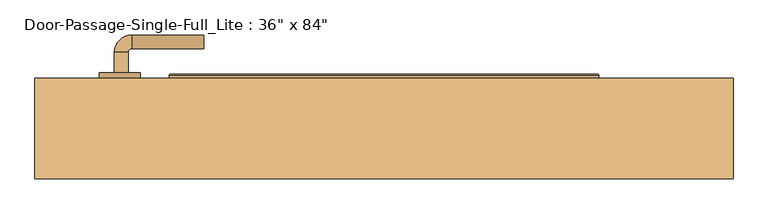
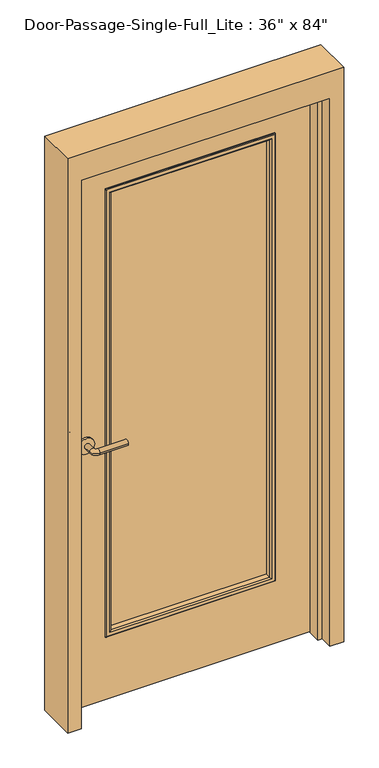
"""IFC4 building model written with IfcOpenShell, lengths in millimetres: door geometry."""

from ifc_helpers import new_model, si_unit, point, frame, frame_2d, origin, place, context, project, spatial, polyline, circle_curve, ellipse_curve, trimmed, segment, composite_curve, outline, extrude, faceted_brep, source, transform, mapped, element, save
from ifc_brep_helpers import plane_surface, cylinder_surface, revolved_surface, advanced_brep


def door_4a7c4c71(model_context):
    return source(origin(), model_context, "Body", "SolidModel", [
        advanced_brep(
        [(-392.190625, 23.75, 1016.0), (-372.190625, 23.75, 1016.0), (-372.190625, -6.25, 1016.0), (-392.190625, -6.25, 1016.0), (-367.190625, -11.25, 1016.0), (-367.190625, -31.25, 1016.0), (-262.190625, -31.25, 1016.0), (-262.190625, -11.25, 1016.0)],
        [
            (0, 1, circle_curve(frame((-382.190625, 23.75, 1016.0), z_axis=(0.0, 1.0, 0.0), x_axis=(1.0, 0.0, 0.0)), 10.0)),
            (1, 0, circle_curve(frame((-382.190625, 23.75, 1016.0), z_axis=(0.0, 1.0, 0.0), x_axis=(1.0, 0.0, 0.0)), 10.0)),
            (1, 2),
            (2, 3, circle_curve(frame((-382.190625, -6.25, 1016.0), z_axis=(0.0, 1.0, 0.0), x_axis=(1.0, 0.0, 0.0)), 10.0)),
            (3, 0),
            (3, 2, circle_curve(frame((-382.190625, -6.25, 1016.0), z_axis=(0.0, 1.0, 0.0), x_axis=(1.0, 0.0, 0.0)), 10.0)),
            (4, 5, circle_curve(frame((-367.190625, -21.25, 1016.0), z_axis=(-1.0, 0.0, 0.0), x_axis=(0.0, 1.0, 0.0)), 10.0)),
            (5, 3, circle_curve(frame((-367.190625, -6.25, 1016.0), z_axis=(0.0, 0.0, -1.0), x_axis=(-1.0, 0.0, 0.0)), 25.0)),
            (2, 4, circle_curve(frame((-367.190625, -6.25, 1016.0), z_axis=(0.0, 0.0, 1.0), x_axis=(-1.0, 0.0, 0.0)), 5.0)),
            (5, 4, circle_curve(frame((-367.190625, -21.25, 1016.0), z_axis=(-1.0, 0.0, 0.0), x_axis=(0.0, 1.0, 0.0)), 10.0)),
            (6, 7, circle_curve(frame((-262.190625, -21.25, 1016.0), z_axis=(1.0, 0.0, 0.0), x_axis=(0.0, 1.0, 0.0)), 10.0)),
            (7, 6, circle_curve(frame((-262.190625, -21.25, 1016.0), z_axis=(1.0, 0.0, 0.0), x_axis=(0.0, 1.0, 0.0)), 10.0)),
            (4, 7),
            (6, 5),
        ],
        [
            plane_surface(frame((-382.190625, 23.75, 1016.0), z_axis=(0.0, 1.0, 0.0), x_axis=(0.0, 0.0, 1.0))),
            cylinder_surface(frame((-382.190625, 23.75, 1016.0), z_axis=(0.0, 1.0, 0.0), x_axis=(1.0, 0.0, 0.0)), 10.0),
            revolved_surface(trimmed(ellipse_curve(frame((-382.190625, -6.25, 1016.0), z_axis=(0.0, -1.0, 0.0), x_axis=(1.0, 0.0, 0.0)), 10.0, 10.0), [point((-392.190625, -6.25, 1016.0))], [point((-372.190625, -6.25, 1016.0))], True, "CARTESIAN"), (-367.190625, -6.25, 1016.0), (0.0, 0.0, -1.0)),
            revolved_surface(trimmed(ellipse_curve(frame((-382.190625, -6.25, 1016.0), z_axis=(0.0, -1.0, 0.0), x_axis=(1.0, 0.0, 0.0)), 10.0, 10.0), [point((-372.190625, -6.25, 1016.0))], [point((-392.190625, -6.25, 1016.0))], True, "CARTESIAN"), (-367.190625, -6.25, 1016.0), (0.0, 0.0, -1.0)),
            plane_surface(frame((-262.190625, -21.25, 1016.0), z_axis=(1.0, 0.0, 0.0), x_axis=(0.0, 0.0, 1.0))),
            cylinder_surface(frame((-367.190625, -21.25, 1016.0), z_axis=(-1.0, 0.0, 0.0), x_axis=(0.0, 1.0, 0.0)), 10.0),
        ],
        [
            (0, [[1, 2]]),
            (1, [[3, 4, 5, -2]]),
            (1, [[-5, 6, -3, -1]]),
            (2, [[7, 8, -4, 9]]),
            (3, [[10, -9, -6, -8]]),
            (4, [[11, 12]]),
            (5, [[13, -11, 14, -7]]),
            (5, [[-14, -12, -13, -10]]),
        ],
    ),
        extrude(outline(composite_curve([segment(trimmed(circle_curve(frame_2d((1016.0, -384.690625)), 30.0), [point((1016.0, -414.690625))], [point((1016.0, -354.690625))], False, "CARTESIAN"), True, "CONTINUOUS"), segment(trimmed(circle_curve(frame_2d((1016.0, -384.690625)), 30.0), [point((1016.0, -354.690625))], [point((1016.0, -414.690625))], False, "CARTESIAN"), True, "CONTINUOUS")], self_intersect=False)), frame((0.0, 23.75, 0.0), z_axis=(0.0, 1.0, 0.0), x_axis=(0.0, 0.0, 1.0)), (0.0, 0.0, 1.0), 8.0),
        advanced_brep(
        [(-392.190625, 84.2, 1016.0), (-372.190625, 84.2, 1016.0), (-392.190625, 114.2, 1016.0), (-372.190625, 114.2, 1016.0), (-367.190625, 119.2, 1016.0), (-367.190625, 139.2, 1016.0), (-262.190625, 139.2, 1016.0), (-262.190625, 119.2, 1016.0)],
        [
            (0, 1, circle_curve(frame((-382.190625, 84.2, 1016.0), z_axis=(0.0, -1.0, 0.0), x_axis=(1.0, 0.0, 0.0)), 10.0)),
            (1, 0, circle_curve(frame((-382.190625, 84.2, 1016.0), z_axis=(0.0, -1.0, 0.0), x_axis=(1.0, 0.0, 0.0)), 10.0)),
            (0, 2),
            (2, 3, circle_curve(frame((-382.190625, 114.2, 1016.0), z_axis=(0.0, -1.0, 0.0), x_axis=(1.0, 0.0, 0.0)), 10.0)),
            (3, 1),
            (3, 2, circle_curve(frame((-382.190625, 114.2, 1016.0), z_axis=(0.0, -1.0, 0.0), x_axis=(1.0, 0.0, 0.0)), 10.0)),
            (4, 3, circle_curve(frame((-367.190625, 114.2, 1016.0), z_axis=(0.0, 0.0, 1.0), x_axis=(-1.0, 0.0, 0.0)), 5.0)),
            (2, 5, circle_curve(frame((-367.190625, 114.2, 1016.0), z_axis=(0.0, 0.0, -1.0), x_axis=(-1.0, 0.0, 0.0)), 25.0)),
            (5, 4, circle_curve(frame((-367.190625, 129.2, 1016.0), z_axis=(-1.0, 0.0, 0.0), x_axis=(0.0, -1.0, 0.0)), 10.0)),
            (4, 5, circle_curve(frame((-367.190625, 129.2, 1016.0), z_axis=(-1.0, 0.0, 0.0), x_axis=(0.0, -1.0, 0.0)), 10.0)),
            (6, 7, circle_curve(frame((-262.190625, 129.2, 1016.0), z_axis=(1.0, 0.0, 0.0), x_axis=(0.0, -1.0, 0.0)), 10.0)),
            (7, 6, circle_curve(frame((-262.190625, 129.2, 1016.0), z_axis=(1.0, 0.0, 0.0), x_axis=(0.0, -1.0, 0.0)), 10.0)),
            (5, 6),
            (7, 4),
        ],
        [
            plane_surface(frame((-382.190625, 84.2, 1016.0), z_axis=(0.0, -1.0, 0.0), x_axis=(0.0, 0.0, 1.0))),
            cylinder_surface(frame((-382.190625, 84.2, 1016.0), z_axis=(0.0, -1.0, 0.0), x_axis=(1.0, 0.0, 0.0)), 10.0),
            revolved_surface(trimmed(ellipse_curve(frame((-382.190625, 114.2, 1016.0), z_axis=(0.0, -1.0, 0.0), x_axis=(1.0, 0.0, 0.0)), 10.0, 10.0), [point((-392.190625, 114.2, 1016.0))], [point((-372.190625, 114.2, 1016.0))], True, "CARTESIAN"), (-367.190625, 114.2, 1016.0), (0.0, 0.0, -1.0)),
            revolved_surface(trimmed(ellipse_curve(frame((-382.190625, 114.2, 1016.0), z_axis=(0.0, -1.0, 0.0), x_axis=(1.0, 0.0, 0.0)), 10.0, 10.0), [point((-372.190625, 114.2, 1016.0))], [point((-392.190625, 114.2, 1016.0))], True, "CARTESIAN"), (-367.190625, 114.2, 1016.0), (0.0, 0.0, -1.0)),
            plane_surface(frame((-262.190625, 129.2, 1016.0), z_axis=(1.0, 0.0, 0.0), x_axis=(0.0, 0.0, 1.0))),
            cylinder_surface(frame((-367.190625, 129.2, 1016.0), z_axis=(-1.0, 0.0, 0.0), x_axis=(0.0, -1.0, 0.0)), 10.0),
        ],
        [
            (0, [[1, 2]]),
            (1, [[-1, 3, 4, 5]]),
            (1, [[-2, -5, 6, -3]]),
            (2, [[7, -4, 8, 9]]),
            (3, [[-8, -6, -7, 10]]),
            (4, [[11, 12]]),
            (5, [[-9, 13, -12, 14]]),
            (5, [[-10, -14, -11, -13]]),
        ],
    ),
        extrude(outline(composite_curve([segment(trimmed(circle_curve(frame_2d((1016.0, -384.690625)), 30.0), [point((1016.0, -414.690625))], [point((1016.0, -354.690625))], False, "CARTESIAN"), True, "CONTINUOUS"), segment(trimmed(circle_curve(frame_2d((1016.0, -384.690625)), 30.0), [point((1016.0, -354.690625))], [point((1016.0, -414.690625))], False, "CARTESIAN"), True, "CONTINUOUS")], self_intersect=False)), frame((0.0, 76.2, 0.0), z_axis=(0.0, 1.0, 0.0), x_axis=(0.0, 0.0, 1.0)), (0.0, 0.0, 1.0), 8.0),
        extrude(outline(polyline([(304.8, 50.8), (-304.8, 50.8), (-304.8, 57.15), (304.8, 57.15), (304.8, 50.8)])), frame((0.0, 0.0, 254.0), z_axis=(0.0, 0.0, 1.0), x_axis=(1.0, 0.0, 0.0)), (0.0, 0.0, 1.0), 1727.2),
        faceted_brep([(457.2, 26.9875, 0.0), (457.2, 76.2, 0.0), (508.0, 76.2, 0.0), (508.0, -69.85, 0.0), (457.2, -69.85, 0.0), (457.2, -20.6375, 0.0), (441.325, -20.6375, 0.0), (441.325, 26.9875, 0.0), (457.2, 26.9875, 2133.6), (457.2, 76.2, 2133.6), (-457.2, 76.2, 2133.6), (-457.2, 76.2, 0.0), (-508.0, 76.2, 0.0), (-508.0, 76.2, 2235.2), (508.0, 76.2, 2235.2), (508.0, -69.85, 2235.2), (-508.0, -69.85, 2235.2), (-508.0, -69.85, 0.0), (-457.2, -69.85, 0.0), (-457.2, -69.85, 2133.6), (457.2, -69.85, 2133.6), (457.2, -20.6375, 2133.6), (-457.2, -20.6375, 2133.6), (-457.2, -20.6375, 0.0), (-441.325, -20.6375, 0.0), (-441.325, -20.6375, 2117.725), (441.325, -20.6375, 2117.725), (441.325, 26.9875, 2117.725), (-441.325, 26.9875, 2117.725), (-441.325, 26.9875, 0.0), (-457.2, 26.9875, 0.0), (-457.2, 26.9875, 2133.6)], [[[0, 1, 2, 3, 4, 5, 6, 7]], [[1, 0, 8, 9]], [[2, 1, 9, 10, 11, 12, 13, 14]], [[3, 2, 14, 15]], [[4, 3, 15, 16, 17, 18, 19, 20]], [[5, 4, 20, 21]], [[6, 5, 21, 22, 23, 24, 25, 26]], [[7, 6, 26, 27]], [[0, 7, 27, 28, 29, 30, 31, 8]], [[9, 8, 31, 10]], [[20, 19, 22, 21]], [[26, 25, 28, 27]], [[12, 11, 30, 29, 24, 23, 18, 17]], [[11, 10, 31, 30]], [[13, 12, 17, 16]], [[19, 18, 23, 22]], [[25, 24, 29, 28]], [[15, 14, 13, 16]]]),
        extrude(outline(polyline([(2133.6, -457.2), (0.0, -457.2), (0.0, 457.2), (2133.6, 457.2), (2133.6, -457.2)]), holes=[polyline([(1981.2, -304.8), (1981.2, 304.8), (254.0, 304.8), (254.0, -304.8), (1981.2, -304.8)])]), frame((0.0, 31.75, 0.0), z_axis=(0.0, 1.0, 0.0), x_axis=(0.0, 0.0, 1.0)), (0.0, 0.0, 1.0), 44.45),
        advanced_brep(
        [(-304.8, 57.15, 1981.2), (-304.8, 76.2, 1981.2), (-304.8, 76.2, 254.0), (-304.8, 57.15, 254.0), (-292.8, 77.2, 1969.2), (-292.8, 57.15, 1969.2), (-292.8, 57.15, 266.0), (-292.8, 77.2, 266.0), (-297.8, 82.2, 1974.2), (-297.8, 82.2, 261.0), (-312.8, 80.2, 1989.2), (-310.8, 82.2, 1987.2), (-310.8, 82.2, 248.0), (-312.8, 80.2, 246.0), (-312.8, 76.2, 1989.2), (-312.8, 76.2, 246.0), (304.8, 76.2, 254.0), (304.8, 57.15, 254.0), (292.8, 57.15, 266.0), (292.8, 77.2, 266.0), (297.8, 82.2, 261.0), (310.8, 82.2, 248.0), (312.8, 80.2, 246.0), (312.8, 76.2, 246.0), (304.8, 76.2, 1981.2), (304.8, 57.15, 1981.2), (292.8, 57.15, 1969.2), (292.8, 77.2, 1969.2), (297.8, 82.2, 1974.2), (310.8, 82.2, 1987.2), (312.8, 80.2, 1989.2), (312.8, 76.2, 1989.2)],
        [
            (0, 1),
            (1, 2),
            (2, 3),
            (3, 0),
            (4, 5),
            (5, 6),
            (6, 7),
            (7, 4),
            (8, 4, ellipse_curve(frame((-297.8, 77.2, 1974.2), z_axis=(-0.7071067811865475, 0.0, -0.7071067811865475), x_axis=(-0.7071067811865474, 0.0, 0.7071067811865476)), 7.0710678, 5.0)),
            (7, 9, ellipse_curve(frame((-297.8, 77.2, 261.0), z_axis=(-0.7071067811865475, 0.0, 0.7071067811865475), x_axis=(0.7071067811865474, 0.0, 0.7071067811865476)), 7.0710678, 5.0)),
            (9, 8),
            (10, 11, ellipse_curve(frame((-310.8, 80.2, 1987.2), z_axis=(-0.7071067811865475, 0.0, -0.7071067811865475), x_axis=(-0.7071067811865474, 0.0, 0.7071067811865476)), 2.8284271, 2.0)),
            (11, 12),
            (12, 13, ellipse_curve(frame((-310.8, 80.2, 248.0), z_axis=(-0.7071067811865475, 0.0, 0.7071067811865475), x_axis=(0.7071067811865474, 0.0, 0.7071067811865476)), 2.8284271, 2.0)),
            (13, 10),
            (14, 10),
            (13, 15),
            (15, 14),
            (2, 16),
            (16, 17),
            (17, 3),
            (6, 18),
            (18, 19),
            (19, 7),
            (19, 20, ellipse_curve(frame((297.8, 77.2, 261.0), z_axis=(-0.7071067811865475, 0.0, -0.7071067811865475), x_axis=(-0.7071067811865476, 0.0, 0.7071067811865474)), 7.0710678, 5.0)),
            (20, 9),
            (12, 21),
            (21, 22, ellipse_curve(frame((310.8, 80.2, 248.0), z_axis=(-0.7071067811865475, 0.0, -0.7071067811865475), x_axis=(-0.7071067811865476, 0.0, 0.7071067811865474)), 2.8284271, 2.0)),
            (22, 13),
            (22, 23),
            (23, 15),
            (16, 24),
            (24, 25),
            (25, 17),
            (18, 26),
            (26, 27),
            (27, 19),
            (27, 28, ellipse_curve(frame((297.8, 77.2, 1974.2), z_axis=(0.7071067811865475, 0.0, -0.7071067811865475), x_axis=(-0.7071067811865474, 0.0, -0.7071067811865476)), 7.0710678, 5.0)),
            (28, 20),
            (21, 29),
            (29, 30, ellipse_curve(frame((310.8, 80.2, 1987.2), z_axis=(0.7071067811865475, 0.0, -0.7071067811865475), x_axis=(-0.7071067811865474, 0.0, -0.7071067811865476)), 2.8284271, 2.0)),
            (30, 22),
            (30, 31),
            (31, 23),
            (31, 14),
            (1, 24),
            (0, 25),
            (5, 26),
            (4, 27),
            (8, 28),
            (11, 29),
            (10, 30),
        ],
        [
            plane_surface(frame((-304.8, 76.2, 1981.2), z_axis=(-1.0, 0.0, 0.0), x_axis=(0.0, 0.0, -1.0))),
            plane_surface(frame((-292.8, 57.15, 1969.2), z_axis=(1.0, 0.0, 0.0), x_axis=(0.0, 0.0, -1.0))),
            cylinder_surface(frame((-297.8, 77.2, 1981.2), z_axis=(0.0, 0.0, 1.0), x_axis=(-1.0, 0.0, 0.0)), 5.0),
            cylinder_surface(frame((-310.8, 80.2, 1981.2), z_axis=(0.0, 0.0, 1.0), x_axis=(-1.0, 0.0, 0.0)), 2.0),
            plane_surface(frame((-312.8, 80.2, 1989.2), z_axis=(-1.0, 0.0, 0.0), x_axis=(0.0, 0.0, -1.0))),
            plane_surface(frame((-304.8, 76.2, 254.0), z_axis=(0.0, 0.0, -1.0), x_axis=(1.0, 0.0, 0.0))),
            plane_surface(frame((-292.8, 57.15, 266.0), z_axis=(0.0, 0.0, 1.0), x_axis=(1.0, 0.0, 0.0))),
            cylinder_surface(frame((-304.8, 77.2, 261.0), z_axis=(-1.0, 0.0, 0.0), x_axis=(0.0, 0.0, -1.0)), 5.0),
            cylinder_surface(frame((-304.8, 80.2, 248.0), z_axis=(-1.0, 0.0, 0.0), x_axis=(0.0, 0.0, -1.0)), 2.0),
            plane_surface(frame((-312.8, 80.2, 246.0), z_axis=(0.0, 0.0, -1.0), x_axis=(1.0, 0.0, 0.0))),
            plane_surface(frame((304.8, 76.2, 254.0), z_axis=(1.0, 0.0, 0.0), x_axis=(0.0, 0.0, 1.0))),
            plane_surface(frame((292.8, 57.15, 266.0), z_axis=(-1.0, 0.0, 0.0), x_axis=(0.0, 0.0, 1.0))),
            cylinder_surface(frame((297.8, 77.2, 254.0), z_axis=(0.0, 0.0, -1.0), x_axis=(1.0, 0.0, 0.0)), 5.0),
            cylinder_surface(frame((310.8, 80.2, 254.0), z_axis=(0.0, 0.0, -1.0), x_axis=(1.0, 0.0, 0.0)), 2.0),
            plane_surface(frame((312.8, 80.2, 246.0), z_axis=(1.0, 0.0, 0.0), x_axis=(0.0, 0.0, 1.0))),
            plane_surface(frame((312.8, 76.2, 1989.2), z_axis=(0.0, -1.0, 0.0), x_axis=(-1.0, 0.0, 0.0))),
            plane_surface(frame((304.8, 76.2, 1981.2), z_axis=(0.0, 0.0, 1.0), x_axis=(-1.0, 0.0, 0.0))),
            plane_surface(frame((304.8, 57.15, 1981.2), z_axis=(0.0, -1.0, 0.0), x_axis=(-1.0, 0.0, 0.0))),
            plane_surface(frame((292.8, 57.15, 1969.2), z_axis=(0.0, 0.0, -1.0), x_axis=(-1.0, 0.0, 0.0))),
            cylinder_surface(frame((304.8, 77.2, 1974.2), z_axis=(1.0, 0.0, 0.0), x_axis=(0.0, 0.0, 1.0)), 5.0),
            plane_surface(frame((297.8, 82.2, 1974.2), z_axis=(0.0, 1.0, 0.0), x_axis=(-1.0, 0.0, 0.0))),
            cylinder_surface(frame((304.8, 80.2, 1987.2), z_axis=(1.0, 0.0, 0.0), x_axis=(0.0, 0.0, 1.0)), 2.0),
            plane_surface(frame((312.8, 80.2, 1989.2), z_axis=(0.0, 0.0, 1.0), x_axis=(-1.0, 0.0, 0.0))),
        ],
        [
            (0, [[1, 2, 3, 4]]),
            (1, [[5, 6, 7, 8]]),
            (2, [[9, -8, 10, 11]]),
            (3, [[12, 13, 14, 15]]),
            (4, [[16, -15, 17, 18]]),
            (5, [[-3, 19, 20, 21]]),
            (6, [[-7, 22, 23, 24]]),
            (7, [[-10, -24, 25, 26]]),
            (8, [[-14, 27, 28, 29]]),
            (9, [[-17, -29, 30, 31]]),
            (10, [[-20, 32, 33, 34]]),
            (11, [[-23, 35, 36, 37]]),
            (12, [[-25, -37, 38, 39]]),
            (13, [[-28, 40, 41, 42]]),
            (14, [[-30, -42, 43, 44]]),
            (15, [[-31, -44, 45, -18], [46, -32, -19, -2]]),
            (16, [[-33, -46, -1, 47]]),
            (17, [[-21, -34, -47, -4], [48, -35, -22, -6]]),
            (18, [[-36, -48, -5, 49]]),
            (19, [[-38, -49, -9, 50]]),
            (20, [[51, -40, -27, -13], [-26, -39, -50, -11]]),
            (21, [[-41, -51, -12, 52]]),
            (22, [[-43, -52, -16, -45]]),
        ],
    ),
        advanced_brep(
        [(-304.8, 50.8, 254.0), (-304.8, 31.75, 254.0), (-304.8, 31.75, 1981.2), (-304.8, 50.8, 1981.2), (-292.8, 30.75, 266.0), (-292.8, 50.8, 266.0), (-292.8, 50.8, 1969.2), (-292.8, 30.75, 1969.2), (-297.8, 25.75, 261.0), (-297.8, 25.75, 1974.2), (-312.8, 27.75, 246.0), (-310.8, 25.75, 248.0), (-310.8, 25.75, 1987.2), (-312.8, 27.75, 1989.2), (-312.8, 31.75, 246.0), (-312.8, 31.75, 1989.2), (304.8, 31.75, 1981.2), (304.8, 50.8, 1981.2), (292.8, 50.8, 1969.2), (292.8, 30.75, 1969.2), (297.8, 25.75, 1974.2), (310.8, 25.75, 1987.2), (312.8, 27.75, 1989.2), (312.8, 31.75, 1989.2), (304.8, 31.75, 254.0), (304.8, 50.8, 254.0), (292.8, 50.8, 266.0), (292.8, 30.75, 266.0), (297.8, 25.75, 261.0), (310.8, 25.75, 248.0), (312.8, 27.75, 246.0), (312.8, 31.75, 246.0)],
        [
            (0, 1),
            (1, 2),
            (2, 3),
            (3, 0),
            (4, 5),
            (5, 6),
            (6, 7),
            (7, 4),
            (8, 4, ellipse_curve(frame((-297.8, 30.75, 261.0), z_axis=(-0.7071067811865475, 0.0, 0.7071067811865475), x_axis=(-0.7071067811865474, 0.0, -0.7071067811865476)), 7.0710678, 5.0)),
            (7, 9, ellipse_curve(frame((-297.8, 30.75, 1974.2), z_axis=(-0.7071067811865475, 0.0, -0.7071067811865475), x_axis=(0.7071067811865474, 0.0, -0.7071067811865476)), 7.0710678, 5.0)),
            (9, 8),
            (10, 11, ellipse_curve(frame((-310.8, 27.75, 248.0), z_axis=(-0.7071067811865475, 0.0, 0.7071067811865475), x_axis=(-0.7071067811865474, 0.0, -0.7071067811865476)), 2.8284271, 2.0)),
            (11, 12),
            (12, 13, ellipse_curve(frame((-310.8, 27.75, 1987.2), z_axis=(-0.7071067811865475, 0.0, -0.7071067811865475), x_axis=(0.7071067811865474, 0.0, -0.7071067811865476)), 2.8284271, 2.0)),
            (13, 10),
            (14, 10),
            (13, 15),
            (15, 14),
            (2, 16),
            (16, 17),
            (17, 3),
            (6, 18),
            (18, 19),
            (19, 7),
            (19, 20, ellipse_curve(frame((297.8, 30.75, 1974.2), z_axis=(-0.7071067811865475, 0.0, 0.7071067811865475), x_axis=(-0.7071067811865476, 0.0, -0.7071067811865474)), 7.0710678, 5.0)),
            (20, 9),
            (12, 21),
            (21, 22, ellipse_curve(frame((310.8, 27.75, 1987.2), z_axis=(-0.7071067811865475, 0.0, 0.7071067811865475), x_axis=(-0.7071067811865476, 0.0, -0.7071067811865474)), 2.8284271, 2.0)),
            (22, 13),
            (22, 23),
            (23, 15),
            (16, 24),
            (24, 25),
            (25, 17),
            (18, 26),
            (26, 27),
            (27, 19),
            (27, 28, ellipse_curve(frame((297.8, 30.75, 261.0), z_axis=(0.7071067811865475, 0.0, 0.7071067811865475), x_axis=(-0.7071067811865474, 0.0, 0.7071067811865476)), 7.0710678, 5.0)),
            (28, 20),
            (21, 29),
            (29, 30, ellipse_curve(frame((310.8, 27.75, 248.0), z_axis=(0.7071067811865475, 0.0, 0.7071067811865475), x_axis=(-0.7071067811865474, 0.0, 0.7071067811865476)), 2.8284271, 2.0)),
            (30, 22),
            (30, 31),
            (31, 23),
            (31, 14),
            (1, 24),
            (0, 25),
            (5, 26),
            (4, 27),
            (8, 28),
            (11, 29),
            (10, 30),
        ],
        [
            plane_surface(frame((-304.8, 31.75, 254.0), z_axis=(-1.0, 0.0, 0.0), x_axis=(0.0, 0.0, 1.0))),
            plane_surface(frame((-292.8, 50.8, 266.0), z_axis=(1.0, 0.0, 0.0), x_axis=(0.0, 0.0, 1.0))),
            cylinder_surface(frame((-297.8, 30.75, 254.0), z_axis=(0.0, 0.0, -1.0), x_axis=(-1.0, 0.0, 0.0)), 5.0),
            cylinder_surface(frame((-310.8, 27.75, 254.0), z_axis=(0.0, 0.0, -1.0), x_axis=(-1.0, 0.0, 0.0)), 2.0),
            plane_surface(frame((-312.8, 27.75, 246.0), z_axis=(-1.0, 0.0, 0.0), x_axis=(0.0, 0.0, 1.0))),
            plane_surface(frame((-304.8, 31.75, 1981.2), z_axis=(0.0, 0.0, 1.0), x_axis=(1.0, 0.0, 0.0))),
            plane_surface(frame((-292.8, 50.8, 1969.2), z_axis=(0.0, 0.0, -1.0), x_axis=(1.0, 0.0, 0.0))),
            cylinder_surface(frame((-304.8, 30.75, 1974.2), z_axis=(-1.0, 0.0, 0.0), x_axis=(0.0, 0.0, 1.0)), 5.0),
            cylinder_surface(frame((-304.8, 27.75, 1987.2), z_axis=(-1.0, 0.0, 0.0), x_axis=(0.0, 0.0, 1.0)), 2.0),
            plane_surface(frame((-312.8, 27.75, 1989.2), z_axis=(0.0, 0.0, 1.0), x_axis=(1.0, 0.0, 0.0))),
            plane_surface(frame((304.8, 31.75, 1981.2), z_axis=(1.0, 0.0, 0.0), x_axis=(0.0, 0.0, -1.0))),
            plane_surface(frame((292.8, 50.8, 1969.2), z_axis=(-1.0, 0.0, 0.0), x_axis=(0.0, 0.0, -1.0))),
            cylinder_surface(frame((297.8, 30.75, 1981.2), z_axis=(0.0, 0.0, 1.0), x_axis=(1.0, 0.0, 0.0)), 5.0),
            cylinder_surface(frame((310.8, 27.75, 1981.2), z_axis=(0.0, 0.0, 1.0), x_axis=(1.0, 0.0, 0.0)), 2.0),
            plane_surface(frame((312.8, 27.75, 1989.2), z_axis=(1.0, 0.0, 0.0), x_axis=(0.0, 0.0, -1.0))),
            plane_surface(frame((312.8, 31.75, 246.0), z_axis=(0.0, 1.0, 0.0), x_axis=(-1.0, 0.0, 0.0))),
            plane_surface(frame((304.8, 31.75, 254.0), z_axis=(0.0, 0.0, -1.0), x_axis=(-1.0, 0.0, 0.0))),
            plane_surface(frame((304.8, 50.8, 254.0), z_axis=(0.0, 1.0, 0.0), x_axis=(-1.0, 0.0, 0.0))),
            plane_surface(frame((292.8, 50.8, 266.0), z_axis=(0.0, 0.0, 1.0), x_axis=(-1.0, 0.0, 0.0))),
            cylinder_surface(frame((304.8, 30.75, 261.0), z_axis=(1.0, 0.0, 0.0), x_axis=(0.0, 0.0, -1.0)), 5.0),
            plane_surface(frame((297.8, 25.75, 261.0), z_axis=(0.0, -1.0, 0.0), x_axis=(-1.0, 0.0, 0.0))),
            cylinder_surface(frame((304.8, 27.75, 248.0), z_axis=(1.0, 0.0, 0.0), x_axis=(0.0, 0.0, -1.0)), 2.0),
            plane_surface(frame((312.8, 27.75, 246.0), z_axis=(0.0, 0.0, -1.0), x_axis=(-1.0, 0.0, 0.0))),
        ],
        [
            (0, [[1, 2, 3, 4]]),
            (1, [[5, 6, 7, 8]]),
            (2, [[9, -8, 10, 11]]),
            (3, [[12, 13, 14, 15]]),
            (4, [[16, -15, 17, 18]]),
            (5, [[-3, 19, 20, 21]]),
            (6, [[-7, 22, 23, 24]]),
            (7, [[-10, -24, 25, 26]]),
            (8, [[-14, 27, 28, 29]]),
            (9, [[-17, -29, 30, 31]]),
            (10, [[-20, 32, 33, 34]]),
            (11, [[-23, 35, 36, 37]]),
            (12, [[-25, -37, 38, 39]]),
            (13, [[-28, 40, 41, 42]]),
            (14, [[-30, -42, 43, 44]]),
            (15, [[-31, -44, 45, -18], [46, -32, -19, -2]]),
            (16, [[-33, -46, -1, 47]]),
            (17, [[-21, -34, -47, -4], [48, -35, -22, -6]]),
            (18, [[-36, -48, -5, 49]]),
            (19, [[-38, -49, -9, 50]]),
            (20, [[51, -40, -27, -13], [-26, -39, -50, -11]]),
            (21, [[-41, -51, -12, 52]]),
            (22, [[-43, -52, -16, -45]]),
        ],
    ),
    ])


if __name__ == "__main__":
    model = new_model("IFC4")
    model_context = context("Model", 3, world=origin())
    ifc_project = project(units=[si_unit("LENGTHUNIT", "METRE", prefix="MILLI")], contexts=[model_context])
    site = spatial("IfcSite", under=ifc_project)
    building = spatial("IfcBuilding", under=site)
    placement = place(None, origin())
    door_shape = door_4a7c4c71(model_context)
    element("IfcDoor", 1, ObjectType="Door-Passage-Single-Full_Lite : 36\" x 84\"", at=placement, inside=building, context=model_context, shape_type="MappedRepresentation", body=[
        mapped(door_shape, transform((0.0, 0.0, 0.0), x_axis=(1.0, 0.0, 0.0), y_axis=(0.0, 1.0, 0.0), z_axis=(0.0, 0.0, 1.0))),
    ])
    save(model, "model.ifc")

# Revit data of these elements
# Type "Door-Passage-Single-Full_Lite : 36\" x 84\""
#   Type Mark = "52"
#   Assembly Code = "B2030100"
#   Analytic Construction = "Wooden"
#   Thickness = 0' - 1 3/4"
#   Thermal Resistance (R) = 2.5876 (h·ft²·°F)/BTU
#   Swing Angle [instance default] = 90.00°
#   Strike Height = 3' - 4"
#   Rough Width [instance default] = 3' - 4"
#   Rough Height [instance default] = 7' - 4"
#   MF Opening Height [instance default] = 0' - 4"
#   MF Opening Width [instance default] = 0' - 4"
#   Inset Calculate [instance default] = 0' - 4"
#   Masonry Inset [instance default] = 0' - 1"
#   Height = 7' - 0"
#   Width = 3' - 0"
#   Heat Transfer Coefficient (U) = 0.3865 BTU/(h·ft²·°F)
#   Masonry Frame Depth = 0' - 5 3/4"
#   Masonry Frame [instance default] = yes
#   Function = 1
#   Dry Wall Frame [instance default] = no
#   Panel Material = Wood - Birch
#   Glazing = Glass
#   Glass Stop Material = Metal - Paint Finish - Grey
#   Frame Material = Metal - Paint Finish - Grey
#   Door Handle Material = Aluminum
#   Visual Light Transmittance = 0
#   Solar Heat Gain Coefficient = 0
#   Wall Closure = (empty or 0)
# Element 1 (IfcDoor, "Door-Passage-Single-Full_Lite : 36\" x 84\"")
#   Inset Calculate = 0' - 3"
#   Masonry Inset = 0' - 0"
#   Materials on its faces: "Metal - Paint Finish - Grey", "Aluminum", "Wood - Birch", "Glass"
# Materials
#   "Wood - Birch": class "Wood", colour RGB 166 116 52, transparency 0, Cost = 0
#   "Glass": class "Glass", colour RGB 0 128 192, transparency 0.75, Description = "Soda Lime Glass", Cost = 0
#   "Metal - Paint Finish - Grey": class "Paint", colour RGB 104 104 104, transparency 0, Cost = 0
#   "Aluminum": class "Metal", colour RGB 247 247 247, transparency 0, Description = "Aluminum 6061", Cost = 0
